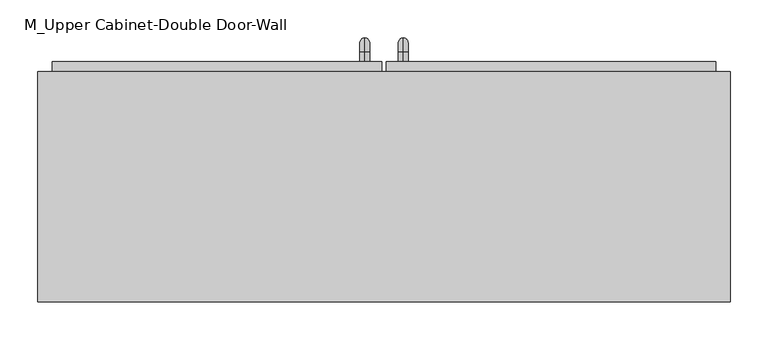
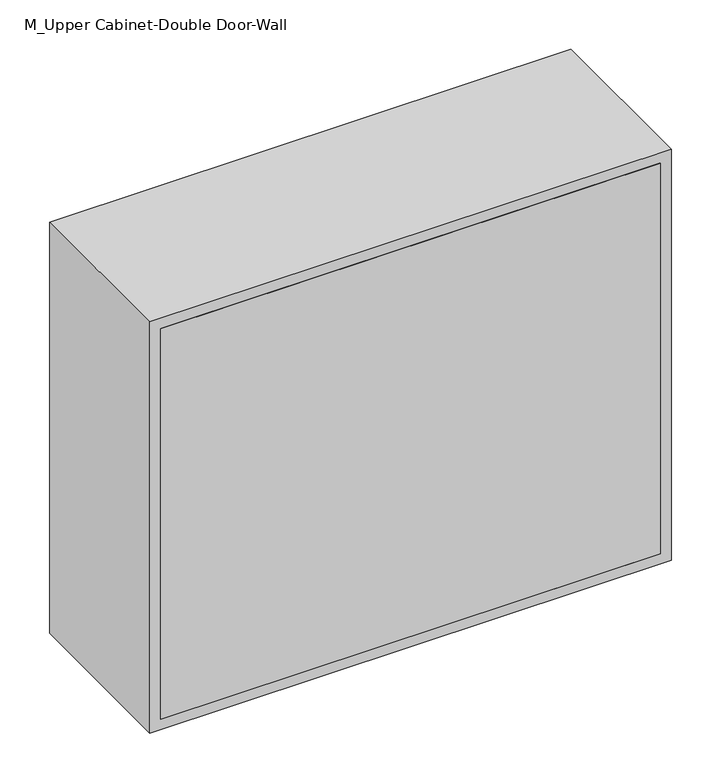
"""IFC4 building model written with IfcOpenShell, lengths in millimetres: furniture geometry, M_Upper Cabinet-Double Door-Wall : 30W X 30H 2."""

from ifc_helpers import new_model, si_unit, point, frame, origin, place, context, project, spatial, polyline, circle_curve, ellipse_curve, trimmed, outline, extrude, source, transform, mapped, element, save
from ifc_brep_helpers import plane_surface, cylinder_surface, revolved_surface, advanced_brep


def m_upper_cabinet_double_door_wall_d1c4bd2f(model_context):
    return source(origin(), model_context, "Body", "SolidModel", [
        advanced_brep(
        [(55.1711628, 393.7, 1212.85), (55.1711628, 393.7, 1225.55), (55.1711628, 406.4, 1212.85), (55.1711628, 406.4, 1225.55), (55.1711628, 425.45, 1206.5), (55.1711628, 412.75, 1206.5), (55.1711628, 412.75, 1130.3), (55.1711628, 425.45, 1130.3), (55.1711628, 406.4, 1111.25), (55.1711628, 406.4, 1123.95), (55.1711628, 393.7, 1123.95), (55.1711628, 393.7, 1111.25)],
        [
            (0, 1, circle_curve(frame((55.1711628, 393.7, 1219.2), z_axis=(0.0, -1.0, 0.0), x_axis=(0.0, 0.0, -1.0)), 6.35)),
            (1, 0, circle_curve(frame((55.1711628, 393.7, 1219.2), z_axis=(0.0, -1.0, 0.0), x_axis=(0.0, 0.0, -1.0)), 6.35)),
            (0, 2),
            (2, 3, circle_curve(frame((55.1711628, 406.4, 1219.2), z_axis=(0.0, -1.0, 0.0), x_axis=(0.0, 0.0, -1.0)), 6.35)),
            (3, 1),
            (3, 2, circle_curve(frame((55.1711628, 406.4, 1219.2), z_axis=(0.0, -1.0, 0.0), x_axis=(0.0, 0.0, -1.0)), 6.35)),
            (4, 3, circle_curve(frame((55.1711628, 406.4, 1206.5), z_axis=(1.0, 0.0, 0.0), x_axis=(0.0, 0.0, 1.0)), 19.05)),
            (2, 5, circle_curve(frame((55.1711628, 406.4, 1206.5), z_axis=(-1.0, 0.0, 0.0), x_axis=(0.0, 0.0, 1.0)), 6.35)),
            (5, 4, circle_curve(frame((55.1711628, 419.1, 1206.5), z_axis=(0.0, 0.0, 1.0), x_axis=(0.0, -1.0, 0.0)), 6.35)),
            (4, 5, circle_curve(frame((55.1711628, 419.1, 1206.5), z_axis=(0.0, 0.0, 1.0), x_axis=(0.0, -1.0, 0.0)), 6.35)),
            (5, 6),
            (6, 7, circle_curve(frame((55.1711628, 419.1, 1130.3), z_axis=(0.0, 0.0, 1.0), x_axis=(0.0, -1.0, 0.0)), 6.35)),
            (7, 4),
            (7, 6, circle_curve(frame((55.1711628, 419.1, 1130.3), z_axis=(0.0, 0.0, 1.0), x_axis=(0.0, -1.0, 0.0)), 6.35)),
            (8, 7, circle_curve(frame((55.1711628, 406.4, 1130.3), z_axis=(1.0, 0.0, 0.0), x_axis=(0.0, 1.0, 0.0)), 19.05)),
            (6, 9, circle_curve(frame((55.1711628, 406.4, 1130.3), z_axis=(-1.0, 0.0, 0.0), x_axis=(0.0, 1.0, 0.0)), 6.35)),
            (9, 8, circle_curve(frame((55.1711628, 406.4, 1117.6), z_axis=(0.0, 1.0, 0.0), x_axis=(0.0, 0.0, 1.0)), 6.35)),
            (8, 9, circle_curve(frame((55.1711628, 406.4, 1117.6), z_axis=(0.0, 1.0, 0.0), x_axis=(0.0, 0.0, 1.0)), 6.35)),
            (10, 11, circle_curve(frame((55.1711628, 393.7, 1117.6), z_axis=(0.0, -1.0, 0.0), x_axis=(0.0, 0.0, 1.0)), 6.35)),
            (11, 10, circle_curve(frame((55.1711628, 393.7, 1117.6), z_axis=(0.0, -1.0, 0.0), x_axis=(0.0, 0.0, 1.0)), 6.35)),
            (9, 10),
            (11, 8),
        ],
        [
            plane_surface(frame((48.8211628, 393.7, 1219.2), z_axis=(0.0, -1.0, 0.0), x_axis=(0.0, 0.0, 1.0))),
            cylinder_surface(frame((55.1711628, 393.7, 1219.2), z_axis=(0.0, -1.0, 0.0), x_axis=(0.0, 0.0, -1.0)), 6.35),
            revolved_surface(trimmed(ellipse_curve(frame((55.1711628, 406.4, 1219.2), z_axis=(0.0, -1.0, 0.0), x_axis=(0.0, 0.0, -1.0)), 6.35, 6.35), [point((55.1711628, 406.4, 1212.85))], [point((55.1711628, 406.4, 1225.55))], True, "CARTESIAN"), (55.1711628, 406.4, 1206.5), (-1.0, 0.0, 0.0)),
            revolved_surface(trimmed(ellipse_curve(frame((55.1711628, 406.4, 1219.2), z_axis=(0.0, -1.0, 0.0), x_axis=(0.0, 0.0, -1.0)), 6.35, 6.35), [point((55.1711628, 406.4, 1225.55))], [point((55.1711628, 406.4, 1212.85))], True, "CARTESIAN"), (55.1711628, 406.4, 1206.5), (-1.0, 0.0, 0.0)),
            cylinder_surface(frame((55.1711628, 419.1, 1206.5), z_axis=(0.0, 0.0, 1.0), x_axis=(0.0, -1.0, 0.0)), 6.35),
            revolved_surface(trimmed(ellipse_curve(frame((55.1711628, 419.1, 1130.3), z_axis=(0.0, 0.0, 1.0), x_axis=(0.0, -1.0, 0.0)), 6.35, 6.35), [point((55.1711628, 412.75, 1130.3))], [point((55.1711628, 425.45, 1130.3))], True, "CARTESIAN"), (55.1711628, 406.4, 1130.3), (-1.0, 0.0, 0.0)),
            revolved_surface(trimmed(ellipse_curve(frame((55.1711628, 419.1, 1130.3), z_axis=(0.0, 0.0, 1.0), x_axis=(0.0, -1.0, 0.0)), 6.35, 6.35), [point((55.1711628, 425.45, 1130.3))], [point((55.1711628, 412.75, 1130.3))], True, "CARTESIAN"), (55.1711628, 406.4, 1130.3), (-1.0, 0.0, 0.0)),
            plane_surface(frame((48.8211628, 393.7, 1117.6), z_axis=(0.0, -1.0, 0.0), x_axis=(0.0, 0.0, -1.0))),
            cylinder_surface(frame((55.1711628, 406.4, 1117.6), z_axis=(0.0, 1.0, 0.0), x_axis=(0.0, 0.0, 1.0)), 6.35),
        ],
        [
            (0, [[1, 2]]),
            (1, [[-1, 3, 4, 5]]),
            (1, [[-2, -5, 6, -3]]),
            (2, [[7, -4, 8, 9]]),
            (3, [[-8, -6, -7, 10]]),
            (4, [[-9, 11, 12, 13]]),
            (4, [[-10, -13, 14, -11]]),
            (5, [[15, -12, 16, 17]]),
            (6, [[-16, -14, -15, 18]]),
            (7, [[19, 20]]),
            (8, [[-17, 21, -20, 22]]),
            (8, [[-18, -22, -19, -21]]),
        ],
    ),
        advanced_brep(
        [(4.3711628, 393.7, 1212.85), (4.3711628, 393.7, 1225.55), (4.3711628, 406.4, 1212.85), (4.3711628, 406.4, 1225.55), (4.3711628, 425.45, 1206.5), (4.3711628, 412.75, 1206.5), (4.3711628, 412.75, 1130.3), (4.3711628, 425.45, 1130.3), (4.3711628, 406.4, 1111.25), (4.3711628, 406.4, 1123.95), (4.3711628, 393.7, 1123.95), (4.3711628, 393.7, 1111.25)],
        [
            (0, 1, circle_curve(frame((4.3711628, 393.7, 1219.2), z_axis=(0.0, -1.0, 0.0), x_axis=(0.0, 0.0, 1.0)), 6.35)),
            (1, 0, circle_curve(frame((4.3711628, 393.7, 1219.2), z_axis=(0.0, -1.0, 0.0), x_axis=(0.0, 0.0, 1.0)), 6.35)),
            (0, 2),
            (2, 3, circle_curve(frame((4.3711628, 406.4, 1219.2), z_axis=(0.0, -1.0, 0.0), x_axis=(0.0, 0.0, 1.0)), 6.35)),
            (3, 1),
            (3, 2, circle_curve(frame((4.3711628, 406.4, 1219.2), z_axis=(0.0, -1.0, 0.0), x_axis=(0.0, 0.0, 1.0)), 6.35)),
            (4, 3, circle_curve(frame((4.3711628, 406.4, 1206.5), z_axis=(1.0, 0.0, 0.0), x_axis=(0.0, 0.0, 1.0)), 19.05)),
            (2, 5, circle_curve(frame((4.3711628, 406.4, 1206.5), z_axis=(-1.0, 0.0, 0.0), x_axis=(0.0, 0.0, 1.0)), 6.35)),
            (5, 4, circle_curve(frame((4.3711628, 419.1, 1206.5), z_axis=(0.0, 0.0, 1.0), x_axis=(0.0, 1.0, 0.0)), 6.35)),
            (4, 5, circle_curve(frame((4.3711628, 419.1, 1206.5), z_axis=(0.0, 0.0, 1.0), x_axis=(0.0, 1.0, 0.0)), 6.35)),
            (5, 6),
            (6, 7, circle_curve(frame((4.3711628, 419.1, 1130.3), z_axis=(0.0, 0.0, 1.0), x_axis=(0.0, 1.0, 0.0)), 6.35)),
            (7, 4),
            (7, 6, circle_curve(frame((4.3711628, 419.1, 1130.3), z_axis=(0.0, 0.0, 1.0), x_axis=(0.0, 1.0, 0.0)), 6.35)),
            (8, 7, circle_curve(frame((4.3711628, 406.4, 1130.3), z_axis=(1.0, 0.0, 0.0), x_axis=(0.0, 1.0, 0.0)), 19.05)),
            (6, 9, circle_curve(frame((4.3711628, 406.4, 1130.3), z_axis=(-1.0, 0.0, 0.0), x_axis=(0.0, 1.0, 0.0)), 6.35)),
            (9, 8, circle_curve(frame((4.3711628, 406.4, 1117.6), z_axis=(0.0, 1.0, 0.0), x_axis=(0.0, 0.0, -1.0)), 6.35)),
            (8, 9, circle_curve(frame((4.3711628, 406.4, 1117.6), z_axis=(0.0, 1.0, 0.0), x_axis=(0.0, 0.0, -1.0)), 6.35)),
            (10, 11, circle_curve(frame((4.3711628, 393.7, 1117.6), z_axis=(0.0, -1.0, 0.0), x_axis=(0.0, 0.0, -1.0)), 6.35)),
            (11, 10, circle_curve(frame((4.3711628, 393.7, 1117.6), z_axis=(0.0, -1.0, 0.0), x_axis=(0.0, 0.0, -1.0)), 6.35)),
            (9, 10),
            (11, 8),
        ],
        [
            plane_surface(frame((-1.9788372, 393.7, 1219.2), z_axis=(0.0, -1.0, 0.0), x_axis=(0.0, 0.0, 1.0))),
            cylinder_surface(frame((4.3711628, 393.7, 1219.2), z_axis=(0.0, -1.0, 0.0), x_axis=(0.0, 0.0, 1.0)), 6.35),
            revolved_surface(trimmed(ellipse_curve(frame((4.3711628, 406.4, 1219.2), z_axis=(0.0, -1.0, 0.0), x_axis=(0.0, 0.0, 1.0)), 6.35, 6.35), [point((4.3711628, 406.4, 1212.85))], [point((4.3711628, 406.4, 1225.55))], True, "CARTESIAN"), (4.3711628, 406.4, 1206.5), (-1.0, 0.0, 0.0)),
            revolved_surface(trimmed(ellipse_curve(frame((4.3711628, 406.4, 1219.2), z_axis=(0.0, -1.0, 0.0), x_axis=(0.0, 0.0, 1.0)), 6.35, 6.35), [point((4.3711628, 406.4, 1225.55))], [point((4.3711628, 406.4, 1212.85))], True, "CARTESIAN"), (4.3711628, 406.4, 1206.5), (-1.0, 0.0, 0.0)),
            cylinder_surface(frame((4.3711628, 419.1, 1206.5), z_axis=(0.0, 0.0, 1.0), x_axis=(0.0, 1.0, 0.0)), 6.35),
            revolved_surface(trimmed(ellipse_curve(frame((4.3711628, 419.1, 1130.3), z_axis=(0.0, 0.0, 1.0), x_axis=(0.0, 1.0, 0.0)), 6.35, 6.35), [point((4.3711628, 412.75, 1130.3))], [point((4.3711628, 425.45, 1130.3))], True, "CARTESIAN"), (4.3711628, 406.4, 1130.3), (-1.0, 0.0, 0.0)),
            revolved_surface(trimmed(ellipse_curve(frame((4.3711628, 419.1, 1130.3), z_axis=(0.0, 0.0, 1.0), x_axis=(0.0, 1.0, 0.0)), 6.35, 6.35), [point((4.3711628, 425.45, 1130.3))], [point((4.3711628, 412.75, 1130.3))], True, "CARTESIAN"), (4.3711628, 406.4, 1130.3), (-1.0, 0.0, 0.0)),
            plane_surface(frame((-1.9788372, 393.7, 1117.6), z_axis=(0.0, -1.0, 0.0), x_axis=(0.0, 0.0, -1.0))),
            cylinder_surface(frame((4.3711628, 406.4, 1117.6), z_axis=(0.0, 1.0, 0.0), x_axis=(0.0, 0.0, -1.0)), 6.35),
        ],
        [
            (0, [[1, 2]]),
            (1, [[-1, 3, 4, 5]]),
            (1, [[-2, -5, 6, -3]]),
            (2, [[7, -4, 8, 9]]),
            (3, [[-8, -6, -7, 10]]),
            (4, [[-9, 11, 12, 13]]),
            (4, [[-10, -13, 14, -11]]),
            (5, [[15, -12, 16, 17]]),
            (6, [[-16, -14, -15, 18]]),
            (7, [[19, 20]]),
            (8, [[-17, 21, -20, 22]]),
            (8, [[-18, -22, -19, -21]]),
        ],
    ),
        extrude(outline(polyline([(32.9461628, 393.7), (467.9211628, 393.7), (467.9211628, 361.95), (32.9461628, 361.95), (32.9461628, 393.7)])), frame((0.0, 0.0, 1085.85), z_axis=(0.0, 0.0, 1.0), x_axis=(1.0, 0.0, 0.0)), (0.0, 0.0, 1.0), 723.9),
        extrude(outline(polyline([(-408.3788372, 393.7), (26.5961628, 393.7), (26.5961628, 361.95), (-408.3788372, 361.95), (-408.3788372, 393.7)])), frame((0.0, 0.0, 1085.85), z_axis=(0.0, 0.0, 1.0), x_axis=(1.0, 0.0, 0.0)), (0.0, 0.0, 1.0), 723.9),
        extrude(outline(polyline([(467.9211628, 76.2), (-408.3788372, 76.2), (-408.3788372, 95.25), (467.9211628, 95.25), (467.9211628, 76.2)])), frame((0.0, 0.0, 1085.85), z_axis=(0.0, 0.0, 1.0), x_axis=(1.0, 0.0, 0.0)), (0.0, 0.0, 1.0), 723.9),
        extrude(outline(polyline([(1828.8, -427.4288372), (1066.8, -427.4288372), (1066.8, 486.9711628), (1828.8, 486.9711628), (1828.8, -427.4288372)]), holes=[polyline([(1809.75, -408.3788372), (1809.75, 467.9211628), (1085.85, 467.9211628), (1085.85, -408.3788372), (1809.75, -408.3788372)])]), frame((0.0, 76.2, 0.0), z_axis=(0.0, 1.0, 0.0), x_axis=(0.0, 0.0, 1.0)), (0.0, 0.0, 1.0), 304.8),
    ])


if __name__ == "__main__":
    model = new_model("IFC4")
    model_context = context("Model", 3, world=origin())
    ifc_project = project(units=[si_unit("LENGTHUNIT", "METRE", prefix="MILLI")], contexts=[model_context])
    site = spatial("IfcSite", under=ifc_project)
    building = spatial("IfcBuilding", under=site)
    placement = place(None, origin())
    m_upper_cabinet_double_door_wall_shape = m_upper_cabinet_double_door_wall_d1c4bd2f(model_context)
    element("IfcFurniture", 1, ObjectType="M_Upper Cabinet-Double Door-Wall : 30W X 30H 2", at=placement, inside=building, context=model_context, shape_type="MappedRepresentation", body=[
        mapped(m_upper_cabinet_double_door_wall_shape, transform((0.0, 0.0, 0.0), x_axis=(1.0, 0.0, 0.0), y_axis=(0.0, 1.0, 0.0), z_axis=(0.0, 0.0, 1.0))),
    ])
    save(model, "model.ifc")

# Revit data of these elements
# Type "M_Upper Cabinet-Double Door-Wall : 30W X 30H 2"
#   Depth = 1' - 0"
#   Height = 2' - 6"
#   Top Of Cabinet = 6' - 0"
#   Width = 3' - 0"
#   Cabinet Material = none
#   Door/Drawer Material = none
#   Handle Material = Cabinets - Handles
# Element 1 (IfcFurniture, "M_Upper Cabinet-Double Door-Wall : 30W X 30H 2")
#   Materials on its faces: "MAX HEIGHT OF  COUNTERTOP 34\"", "Cabinets - Handles"
# Materials
#   "Cabinets - Handles": class "Metal", colour RGB 57 57 57, transparency 0
#   "MAX HEIGHT OF  COUNTERTOP 34\"": class "Generic", colour RGB 181 181 181, transparency 0, Cost = 0
